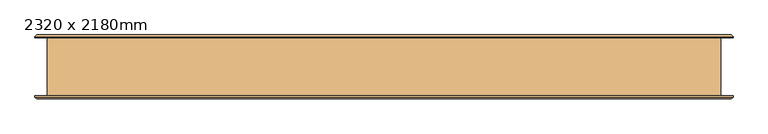
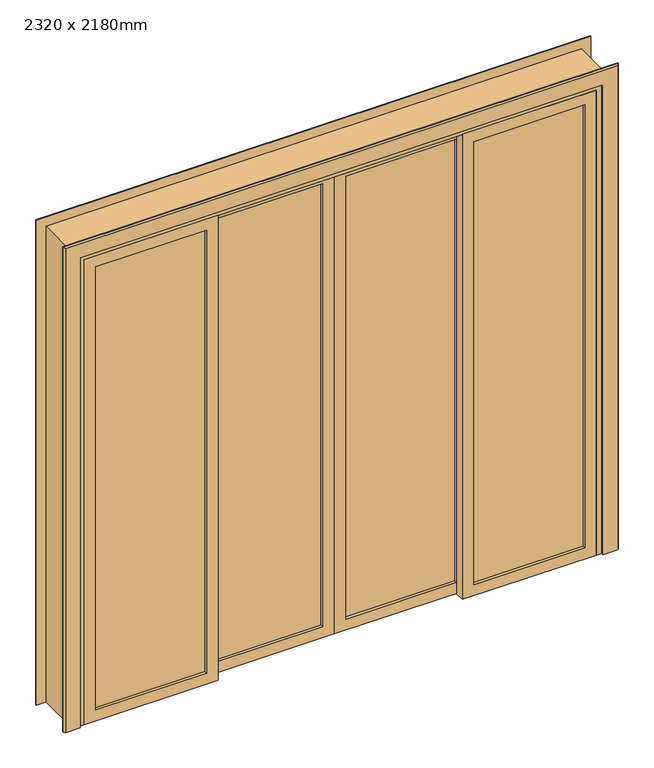
"""IFC4 building model written with IfcOpenShell, lengths in millimetres: door geometry, Porta envidraçada de correr quádrupla com revestimento : 2320 x 2180mm."""

from ifc_helpers import new_model, si_unit, point, frame, frame_2d, origin, place, context, project, spatial, polyline, circle_curve, trimmed, segment, composite_curve, outline, extrude, faceted_brep, source, transform, mapped, element, save


def door_2320_x_2180mm_c20d597c(model_context):
    return source(origin(), model_context, "Body", "SolidModel", [
        extrude(outline(composite_curve([segment(trimmed(circle_curve(frame_2d((990.0, 15.0)), 10.0), [point((1000.0, 15.0))], [point((990.0, 5.0))], False, "CARTESIAN"), True, "CONTINUOUS"), segment(polyline([(990.0, 5.0), (810.0, 5.0)]), True, "CONTINUOUS"), segment(trimmed(circle_curve(frame_2d((810.0, 15.0)), 10.0), [point((810.0, 5.0))], [point((800.0, 15.0))], False, "CARTESIAN"), True, "CONTINUOUS"), segment(polyline([(800.0, 15.0), (800.0, 35.0)]), True, "CONTINUOUS"), segment(trimmed(circle_curve(frame_2d((810.0, 35.0)), 10.0), [point((800.0, 35.0))], [point((810.0, 45.0))], False, "CARTESIAN"), True, "CONTINUOUS"), segment(polyline([(810.0, 45.0), (990.0, 45.0)]), True, "CONTINUOUS"), segment(trimmed(circle_curve(frame_2d((990.0, 35.0)), 10.0), [point((990.0, 45.0))], [point((1000.0, 35.0))], False, "CARTESIAN"), True, "CONTINUOUS"), segment(polyline([(1000.0, 35.0), (1000.0, 15.0)]), True, "CONTINUOUS")], self_intersect=False), holes=[composite_curve([segment(trimmed(circle_curve(frame_2d((985.0, 25.0)), 5.0), [point((985.0, 20.0))], [point((985.0, 30.0))], True, "CARTESIAN"), True, "CONTINUOUS"), segment(trimmed(circle_curve(frame_2d((985.0, 25.0)), 5.0), [point((985.0, 30.0))], [point((985.0, 20.0))], True, "CARTESIAN"), True, "CONTINUOUS")], self_intersect=False), composite_curve([segment(trimmed(circle_curve(frame_2d((815.0, 25.0)), 5.0), [point((815.0, 20.0))], [point((815.0, 30.0))], True, "CARTESIAN"), True, "CONTINUOUS"), segment(trimmed(circle_curve(frame_2d((815.0, 25.0)), 5.0), [point((815.0, 30.0))], [point((815.0, 20.0))], True, "CARTESIAN"), True, "CONTINUOUS")], self_intersect=False), composite_curve([segment(polyline([(960.0, 15.0), (960.0, 35.0)]), True, "CONTINUOUS"), segment(trimmed(circle_curve(frame_2d((955.0, 35.0)), 5.0), [point((960.0, 35.0))], [point((955.0, 40.0))], True, "CARTESIAN"), True, "CONTINUOUS"), segment(polyline([(955.0, 40.0), (845.0, 40.0)]), True, "CONTINUOUS"), segment(trimmed(circle_curve(frame_2d((845.0, 35.0)), 5.0), [point((845.0, 40.0))], [point((840.0, 35.0))], True, "CARTESIAN"), True, "CONTINUOUS"), segment(polyline([(840.0, 35.0), (840.0, 15.0)]), True, "CONTINUOUS"), segment(trimmed(circle_curve(frame_2d((845.0, 15.0)), 5.0), [point((840.0, 15.0))], [point((845.0, 10.0))], True, "CARTESIAN"), True, "CONTINUOUS"), segment(polyline([(845.0, 10.0), (955.0, 10.0)]), True, "CONTINUOUS"), segment(trimmed(circle_curve(frame_2d((955.0, 15.0)), 5.0), [point((955.0, 10.0))], [point((960.0, 15.0))], True, "CARTESIAN"), True, "CONTINUOUS")], self_intersect=False)]), frame((0.0, -15.0, 0.0), z_axis=(0.0, 1.0, 0.0), x_axis=(0.0, 0.0, 1.0)), (0.0, 0.0, 1.0), 3.0),
        extrude(outline(composite_curve([segment(trimmed(circle_curve(frame_2d((990.0, -35.0)), 10.0), [point((1000.0, -35.0))], [point((990.0, -45.0))], False, "CARTESIAN"), True, "CONTINUOUS"), segment(polyline([(990.0, -45.0), (810.0, -45.0)]), True, "CONTINUOUS"), segment(trimmed(circle_curve(frame_2d((810.0, -35.0)), 10.0), [point((810.0, -45.0))], [point((800.0, -35.0))], False, "CARTESIAN"), True, "CONTINUOUS"), segment(polyline([(800.0, -35.0), (800.0, -15.0)]), True, "CONTINUOUS"), segment(trimmed(circle_curve(frame_2d((810.0, -15.0)), 10.0), [point((800.0, -15.0))], [point((810.0, -5.0))], False, "CARTESIAN"), True, "CONTINUOUS"), segment(polyline([(810.0, -5.0), (990.0, -5.0)]), True, "CONTINUOUS"), segment(trimmed(circle_curve(frame_2d((990.0, -15.0)), 10.0), [point((990.0, -5.0))], [point((1000.0, -15.0))], False, "CARTESIAN"), True, "CONTINUOUS"), segment(polyline([(1000.0, -15.0), (1000.0, -35.0)]), True, "CONTINUOUS")], self_intersect=False), holes=[composite_curve([segment(trimmed(circle_curve(frame_2d((985.0, -25.0)), 5.0), [point((985.0, -30.0))], [point((985.0, -20.0))], True, "CARTESIAN"), True, "CONTINUOUS"), segment(trimmed(circle_curve(frame_2d((985.0, -25.0)), 5.0), [point((985.0, -20.0))], [point((985.0, -30.0))], True, "CARTESIAN"), True, "CONTINUOUS")], self_intersect=False), composite_curve([segment(trimmed(circle_curve(frame_2d((815.0, -25.0)), 5.0), [point((815.0, -30.0))], [point((815.0, -20.0))], True, "CARTESIAN"), True, "CONTINUOUS"), segment(trimmed(circle_curve(frame_2d((815.0, -25.0)), 5.0), [point((815.0, -20.0))], [point((815.0, -30.0))], True, "CARTESIAN"), True, "CONTINUOUS")], self_intersect=False), composite_curve([segment(polyline([(960.0, -35.0), (960.0, -15.0)]), True, "CONTINUOUS"), segment(trimmed(circle_curve(frame_2d((955.0, -15.0)), 5.0), [point((960.0, -15.0))], [point((955.0, -10.0))], True, "CARTESIAN"), True, "CONTINUOUS"), segment(polyline([(955.0, -10.0), (845.0, -10.0)]), True, "CONTINUOUS"), segment(trimmed(circle_curve(frame_2d((845.0, -15.0)), 5.0), [point((845.0, -10.0))], [point((840.0, -15.0))], True, "CARTESIAN"), True, "CONTINUOUS"), segment(polyline([(840.0, -15.0), (840.0, -35.0)]), True, "CONTINUOUS"), segment(trimmed(circle_curve(frame_2d((845.0, -35.0)), 5.0), [point((840.0, -35.0))], [point((845.0, -40.0))], True, "CARTESIAN"), True, "CONTINUOUS"), segment(polyline([(845.0, -40.0), (955.0, -40.0)]), True, "CONTINUOUS"), segment(trimmed(circle_curve(frame_2d((955.0, -35.0)), 5.0), [point((955.0, -40.0))], [point((960.0, -35.0))], True, "CARTESIAN"), True, "CONTINUOUS")], self_intersect=False)]), frame((0.0, -15.0, 0.0), z_axis=(0.0, 1.0, 0.0), x_axis=(0.0, 0.0, 1.0)), (0.0, 0.0, 1.0), 3.0),
        extrude(outline(polyline([(2130.0, -580.0), (0.0, -580.0), (0.0, 0.0), (2130.0, 0.0), (2130.0, -580.0)]), holes=[polyline([(2080.0, -50.0), (50.0, -50.0), (50.0, -530.0), (2080.0, -530.0), (2080.0, -50.0)])]), frame((0.0, -55.0, 0.0), z_axis=(0.0, 1.0, 0.0), x_axis=(0.0, 0.0, 1.0)), (0.0, 0.0, 1.0), 40.0),
        extrude(outline(polyline([(2130.0, 530.0), (0.0, 530.0), (0.0, 1110.0), (2130.0, 1110.0), (2130.0, 530.0)]), holes=[polyline([(2080.0, 1060.0), (50.0, 1060.0), (50.0, 580.0), (2080.0, 580.0), (2080.0, 1060.0)])]), frame((0.0, -100.0, 0.0), z_axis=(0.0, 1.0, 0.0), x_axis=(0.0, 0.0, 1.0)), (0.0, 0.0, 1.0), 40.0),
        extrude(outline(polyline([(2130.0, 0.0), (0.0, 0.0), (0.0, 580.0), (2130.0, 580.0), (2130.0, 0.0)]), holes=[polyline([(2080.0, 530.0), (50.0, 530.0), (50.0, 50.0), (2080.0, 50.0), (2080.0, 530.0)])]), frame((0.0, -55.0, 0.0), z_axis=(0.0, 1.0, 0.0), x_axis=(0.0, 0.0, 1.0)), (0.0, 0.0, 1.0), 40.0),
        extrude(outline(polyline([(2130.0, -1110.0), (0.0, -1110.0), (0.0, -530.0), (2130.0, -530.0), (2130.0, -1110.0)]), holes=[polyline([(2080.0, -580.0), (50.0, -580.0), (50.0, -1060.0), (2080.0, -1060.0), (2080.0, -580.0)])]), frame((0.0, -100.0, 0.0), z_axis=(0.0, 1.0, 0.0), x_axis=(0.0, 0.0, 1.0)), (0.0, 0.0, 1.0), 40.0),
        extrude(outline(polyline([(0.0, 1110.0), (0.0, 1160.0), (2180.0, 1160.0), (2180.0, -1160.0), (0.0, -1160.0), (0.0, -1110.0), (2130.0, -1110.0), (2130.0, 1110.0), (0.0, 1110.0)])), frame((0.0, -100.0, 0.0), z_axis=(0.0, 1.0, 0.0), x_axis=(0.0, 0.0, 1.0)), (0.0, 0.0, 1.0), 200.0),
        extrude(outline(polyline([(530.0, -28.0), (530.0, -42.0), (50.0, -42.0), (50.0, -28.0), (530.0, -28.0)])), frame((0.0, 0.0, 50.0), z_axis=(0.0, 0.0, 1.0), x_axis=(1.0, 0.0, 0.0)), (0.0, 0.0, 1.0), 2030.0),
        extrude(outline(polyline([(1060.0, -73.0), (1060.0, -87.0), (580.0, -87.0), (580.0, -73.0), (1060.0, -73.0)])), frame((0.0, 0.0, 50.0), z_axis=(0.0, 0.0, 1.0), x_axis=(1.0, 0.0, 0.0)), (0.0, 0.0, 1.0), 2030.0),
        extrude(outline(polyline([(-580.0, -73.0), (-580.0, -87.0), (-1060.0, -87.0), (-1060.0, -73.0), (-580.0, -73.0)])), frame((0.0, 0.0, 50.0), z_axis=(0.0, 0.0, 1.0), x_axis=(1.0, 0.0, 0.0)), (0.0, 0.0, 1.0), 2030.0),
        extrude(outline(polyline([(-50.0, -28.0), (-50.0, -42.0), (-530.0, -42.0), (-530.0, -28.0), (-50.0, -28.0)])), frame((0.0, 0.0, 50.0), z_axis=(0.0, 0.0, 1.0), x_axis=(1.0, 0.0, 0.0)), (0.0, 0.0, 1.0), 2030.0),
        extrude(outline(polyline([(-580.0, -73.0), (-580.0, -87.0), (-1060.0, -87.0), (-1060.0, -73.0), (-580.0, -73.0)])), frame((0.0, 0.0, 50.0), z_axis=(0.0, 0.0, 1.0), x_axis=(1.0, 0.0, 0.0)), (0.0, 0.0, 1.0), 2030.0),
        extrude(outline(polyline([(-50.0, -28.0), (-50.0, -42.0), (-530.0, -42.0), (-530.0, -28.0), (-50.0, -28.0)])), frame((0.0, 0.0, 50.0), z_axis=(0.0, 0.0, 1.0), x_axis=(1.0, 0.0, 0.0)), (0.0, 0.0, 1.0), 2030.0),
        extrude(outline(polyline([(580.0, -73.0), (1060.0, -73.0), (1060.0, -87.0), (580.0, -87.0), (580.0, -73.0)])), frame((0.0, 0.0, 50.0), z_axis=(0.0, 0.0, 1.0), x_axis=(1.0, 0.0, 0.0)), (0.0, 0.0, 1.0), 2030.0),
        extrude(outline(polyline([(50.0, -28.0), (530.0, -28.0), (530.0, -42.0), (50.0, -42.0), (50.0, -28.0)])), frame((0.0, 0.0, 50.0), z_axis=(0.0, 0.0, 1.0), x_axis=(1.0, 0.0, 0.0)), (0.0, 0.0, 1.0), 2030.0),
        faceted_brep([(1203.0, 104.0, 0.0), (1203.0, 100.0, 0.0), (1133.0, 100.0, 0.0), (1133.0, 110.0, 0.0), (1197.0, 110.0, 0.0), (1203.0, 104.0, 2223.0), (1203.0, 100.0, 2223.0), (-1203.0, 100.0, 2223.0), (-1203.0, 100.0, 0.0), (-1133.0, 100.0, 0.0), (-1133.0, 100.0, 2153.0), (1133.0, 100.0, 2153.0), (1133.0, 110.0, 2153.0), (-1133.0, 110.0, 2153.0), (-1133.0, 110.0, 0.0), (-1197.0, 110.0, 0.0), (-1197.0, 110.0, 2217.0), (1197.0, 110.0, 2217.0), (-1203.0, 104.0, 0.0), (-1203.0, 104.0, 2223.0)], [[[0, 1, 2, 3, 4]], [[1, 0, 5, 6]], [[2, 1, 6, 7, 8, 9, 10, 11]], [[3, 2, 11, 12]], [[4, 3, 12, 13, 14, 15, 16, 17]], [[0, 4, 17, 5]], [[13, 10, 9, 14]], [[18, 15, 14, 9, 8]], [[19, 16, 15, 18]], [[7, 19, 18, 8]], [[5, 17, 16, 19]], [[12, 11, 10, 13]], [[6, 5, 19, 7]]]),
        faceted_brep([(1203.0, -104.0, 0.0), (1197.0, -110.0, 0.0), (1133.0, -110.0, 0.0), (1133.0, -100.0, 0.0), (1203.0, -100.0, 0.0), (1203.0, -104.0, 2223.0), (1197.0, -110.0, 2217.0), (-1197.0, -110.0, 2217.0), (-1197.0, -110.0, 0.0), (-1133.0, -110.0, 0.0), (-1133.0, -110.0, 2153.0), (1133.0, -110.0, 2153.0), (1133.0, -100.0, 2153.0), (-1133.0, -100.0, 2153.0), (-1133.0, -100.0, 0.0), (-1203.0, -100.0, 0.0), (-1203.0, -100.0, 2223.0), (1203.0, -100.0, 2223.0), (-1203.0, -104.0, 2223.0), (-1203.0, -104.0, 0.0)], [[[0, 1, 2, 3, 4]], [[1, 0, 5, 6]], [[2, 1, 6, 7, 8, 9, 10, 11]], [[3, 2, 11, 12]], [[4, 3, 12, 13, 14, 15, 16, 17]], [[0, 4, 17, 5]], [[7, 18, 19, 8]], [[19, 15, 14, 9, 8]], [[13, 10, 9, 14]], [[18, 16, 15, 19]], [[6, 5, 18, 7]], [[12, 11, 10, 13]], [[5, 17, 16, 18]]]),
    ])


if __name__ == "__main__":
    model = new_model("IFC4")
    model_context = context("Model", 3, world=origin())
    ifc_project = project(units=[si_unit("LENGTHUNIT", "METRE", prefix="MILLI")], contexts=[model_context])
    site = spatial("IfcSite", under=ifc_project)
    building = spatial("IfcBuilding", under=site)
    placement = place(None, origin())
    door_2320_x_2180mm_shape = door_2320_x_2180mm_c20d597c(model_context)
    element("IfcDoor", 1, ObjectType="Porta envidraçada de correr quádrupla com revestimento : 2320 x 2180mm", at=placement, inside=building, context=model_context, shape_type="MappedRepresentation", body=[
        mapped(door_2320_x_2180mm_shape, transform((0.0, 0.0, 0.0), x_axis=(1.0, 0.0, 0.0), y_axis=(0.0, 1.0, 0.0), z_axis=(0.0, 0.0, 1.0))),
    ])
    save(model, "model.ifc")

# Revit data of these elements
# Type "Porta envidraçada de correr quádrupla com revestimento : 2320 x 2180mm"
#   Type Mark = "23"
#   Construction Type Id = "GSP4R"
#   Analytic Construction = "Vidraça única Pilkington 1/8 pol"
#   Visual Light Transmittance = 0.9
#   Largura da apara = 70 mm
#   Espessura da apara = 10 mm
#   Solar Heat Gain Coefficient = 0.78
#   Rough Width = 2320 mm
#   Rough Height = 2180 mm
#   Largura da moldura do painel = 50 mm
#   Espessura da moldura do painel = 40 mm
#   Heat Transfer Coefficient (U) = 3.6886 W/(m²·K)
#   Largura do puxador = 40 mm
#   Altura do puxador = 200 mm
#   Largura da estrutura = 50 mm
#   Height = 2180 mm
#   Width = 2320 mm
#   Function = 1
#   Material da apara = none
#   Material do puxador = none
#   Vidro = none
#   Material da moldura = none
#   Thickness = 0
#   Wall Closure = (empty or 0)
# Element 1 (IfcDoor, "Porta envidraçada de correr quádrupla com revestimento : 2320 x 2180mm")
#   Materials on its faces: "Vidro"
# Materials
#   "Vidro": class "Vidro", colour RGB 0 128 192, transparency 0.9, Description = "Vidro de sílica", Cost = 0
